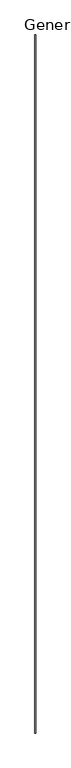
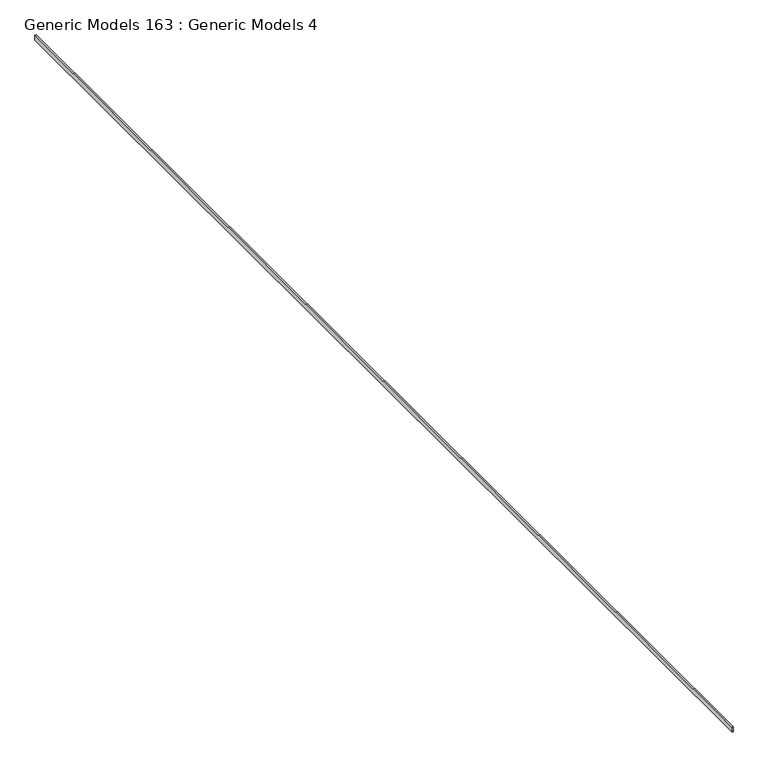
"""IFC4 building model written with IfcOpenShell, lengths in millimetres: proxy geometry, Generic Models 163 : Generic Models 4."""

from ifc_helpers import new_model, si_unit, frame, origin, place, context, project, spatial, polyline, outline, extrude, source, transform, mapped, element, save


def generic_models_163_generic_models_4_489acf9b(model_context):
    return source(origin(), model_context, "Body", "SweptSolid", [
        extrude(outline(polyline([(-10252.9339552, -5493.3230338), (-10252.9339552, 7054.2769662), (-10237.6972239, 7054.2769662), (-10237.6972239, -5493.3230338), (-10252.9339552, -5493.3230338)])), frame((0.0, 0.0, 122784.1984874), z_axis=(0.0, 0.0, 1.0), x_axis=(1.0, 0.0, 0.0)), (0.0, 0.0, 1.0), 54.2029547),
    ])


if __name__ == "__main__":
    model = new_model("IFC4")
    model_context = context("Model", 3, world=origin())
    ifc_project = project(units=[si_unit("LENGTHUNIT", "METRE", prefix="MILLI")], contexts=[model_context])
    site = spatial("IfcSite", under=ifc_project)
    building = spatial("IfcBuilding", under=site)
    placement = place(None, origin())
    generic_models_163_generic_models_4_shape = generic_models_163_generic_models_4_489acf9b(model_context)
    element("IfcBuildingElementProxy", 1, Name="Generic Models 163 : Generic Models 4", ObjectType="Generic Models 163 : Generic Models 4", at=placement, inside=building, context=model_context, shape_type="MappedRepresentation", body=[
        mapped(generic_models_163_generic_models_4_shape, transform((0.0, 0.0, 0.0), x_axis=(1.0, 0.0, 0.0), y_axis=(0.0, 1.0, 0.0), z_axis=(0.0, 0.0, 1.0))),
    ])
    save(model, "model.ifc")

# Revit data of these elements
# Element 1 (IfcBuildingElementProxy, "Generic Models 163 : Generic Models 4")
#   Materials on its faces: "_MORTAR SETTING BED"
# Materials
#   "_MORTAR SETTING BED": class "Generic", colour RGB 191 191 191, transparency 0, Cost = 0
